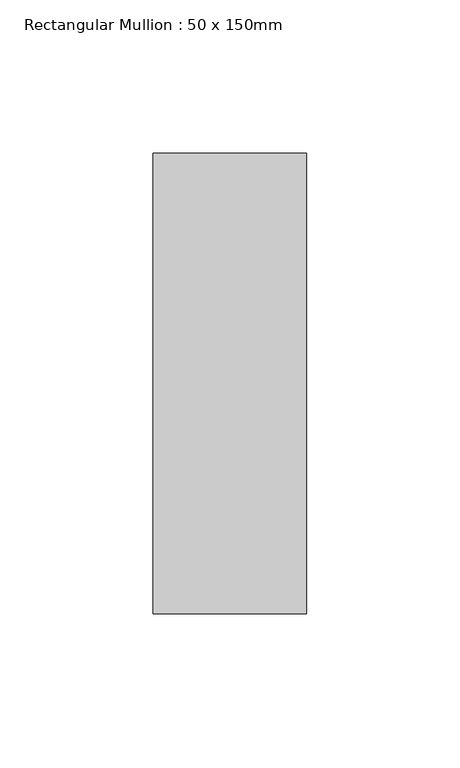
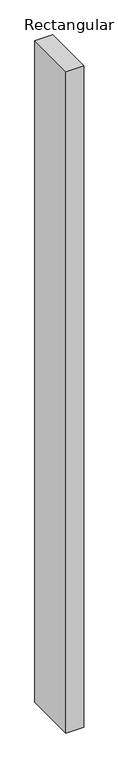
"""IFC4 building model written with IfcOpenShell, lengths in millimetres: member geometry, Rectangular Mullion : 50 x 150mm."""

from ifc_helpers import new_model, si_unit, frame, origin, place, context, project, spatial, polyline, outline, extrude, source, transform, mapped, element, save


def rectangular_mullion_50_x_150mm_f1645b81(model_context):
    return source(origin(), model_context, "Body", "SweptSolid", [
        extrude(outline(polyline([(25.0, 75.0), (25.0, -75.0), (-25.0, -75.0), (-25.0, 75.0), (25.0, 75.0)])), frame((0.0, 0.0, -1950.0000003), z_axis=(0.0, 0.0, 1.0), x_axis=(1.0, 0.0, 0.0)), (0.0, 0.0, 1.0), 1950.0000003),
    ])


if __name__ == "__main__":
    model = new_model("IFC4")
    model_context = context("Model", 3, world=origin())
    ifc_project = project(units=[si_unit("LENGTHUNIT", "METRE", prefix="MILLI")], contexts=[model_context])
    site = spatial("IfcSite", under=ifc_project)
    building = spatial("IfcBuilding", under=site)
    placement = place(None, origin())
    rectangular_mullion_50_x_150mm_shape = rectangular_mullion_50_x_150mm_f1645b81(model_context)
    element("IfcMember", 1, ObjectType="Rectangular Mullion : 50 x 150mm", at=placement, inside=building, context=model_context, shape_type="MappedRepresentation", body=[
        mapped(rectangular_mullion_50_x_150mm_shape, transform((0.0, 0.0, 0.0), x_axis=(1.0, 0.0, 0.0), y_axis=(0.0, 1.0, 0.0), z_axis=(0.0, 0.0, 1.0))),
    ])
    save(model, "model.ifc")

# Revit data of these elements
# Type "Rectangular Mullion : 50 x 150mm"
#   built-in parameter 1007304 = 0.492126 (stored number, unit not read)
#   built-in parameter 1007301 = 0.082021 (stored number, unit not read)
#   built-in parameter 1007300 = 0.082021 (stored number, unit not read)
# Element 1 (IfcMember, "Rectangular Mullion : 50 x 150mm")
#   Materials on its faces: "Metal - Aluminium"
# Materials
#   "Metal - Aluminium": class "Metal", colour RGB 247 247 247, transparency 0
